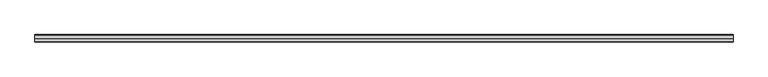
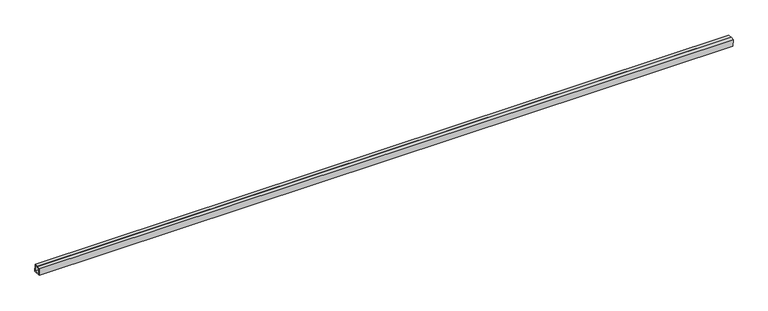
"""IFC4 building model written with IfcOpenShell, lengths in millimetres: proxy geometry, Inner panel:Inner panel:1:Inner panel:1 : Inner panel:Inner panel:300324:2:Inner panel:1:Inner panel:1 : Inner panel:Inner panel:300324:2 : Inner panel:Inner panel:1:Inner panel:1 : Inner panel:Inner panel:300324:300043:20 : Inner panel:Inner panel:1:Inner panel:1 : Inner panel:Inner panel:300324:2:Inner panel:1:Inner panel:1 : Inner panel:Inner panel:300324:2 : Inner panel:Inner panel:1:Inner panel:1 : Inner panel:Inner panel:300324:300043:308120."""

from ifc_helpers import new_model, si_unit, frame, origin, place, context, project, spatial, polyline, outline, extrude, source, transform, mapped, element, save


def generic_models_a2e03578(model_context):
    return source(origin(), model_context, "Body", "SweptSolid", [
        extrude(outline(polyline([(-569061.6758054, 8767.2361869), (-569043.4353822, 8767.9962045), (-569041.8492584, 8729.9292345), (-569079.9162285, 8728.3431107), (-569081.5023523, 8766.4100808), (-569063.2619291, 8767.1700984), (-569063.1627964, 8764.7909128), (-569079.0240339, 8764.1300279), (-569077.6361756, 8730.8214291), (-569044.3275768, 8732.2092874), (-569045.7154351, 8765.5178862), (-569061.5766726, 8764.8570013), (-569061.6758054, 8767.2361869)])), frame((593141.1867242, 0.0, 0.0), z_axis=(1.0, 0.0, 0.0), x_axis=(0.0, 1.0, 0.0)), (0.0, 0.0, 1.0), 3657.6),
    ])


if __name__ == "__main__":
    model = new_model("IFC4")
    model_context = context("Model", 3, world=origin())
    ifc_project = project(units=[si_unit("LENGTHUNIT", "METRE", prefix="MILLI")], contexts=[model_context])
    site = spatial("IfcSite", under=ifc_project)
    building = spatial("IfcBuilding", under=site)
    placement = place(None, origin())
    generic_models_shape = generic_models_a2e03578(model_context)
    element("IfcBuildingElementProxy", 1, Name="Inner panel:Inner panel:1:Inner panel:1 : Inner panel:Inner panel:300324:2:Inner panel:1:Inner panel:1 : Inner panel:Inner panel:300324:2 : Inner panel:Inner panel:1:Inner panel:1 : Inner panel:Inner panel:300324:300043:20 : Inner panel:Inner panel:1:Inner panel:1 : Inner panel:Inner panel:300324:2:Inner panel:1:Inner panel:1 : Inner panel:Inner panel:300324:2 : Inner panel:Inner panel:1:Inner panel:1 : Inner panel:Inner panel:300324:300043:308120", ObjectType="Inner panel:Inner panel:1:Inner panel:1 : Inner panel:Inner panel:300324:2:Inner panel:1:Inner panel:1 : Inner panel:Inner panel:300324:2 : Inner panel:Inner panel:1:Inner panel:1 : Inner panel:Inner panel:300324:300043:20 : Inner panel:Inner panel:1:Inner panel:1 : Inner panel:Inner panel:300324:2:Inner panel:1:Inner panel:1 : Inner panel:Inner panel:300324:2 : Inner panel:Inner panel:1:Inner panel:1 : Inner panel:Inner panel:300324:300043:308120", at=placement, inside=building, context=model_context, shape_type="MappedRepresentation", body=[
        mapped(generic_models_shape, transform((0.0, 0.0, 0.0), x_axis=(1.0, 0.0, 0.0), y_axis=(0.0, 1.0, 0.0), z_axis=(0.0, 0.0, 1.0))),
    ])
    save(model, "model.ifc")

# Revit data of these elements
# Type "Inner panel:Inner panel:1:Inner panel:1 : Inner panel:Inner panel:300324:2:Inner panel:1:Inner panel:1 : Inner panel:Inner panel:300324:2 : Inner panel:Inner panel:1:Inner panel:1 : Inner panel:Inner panel:300324:300043:20 : Inner panel:Inner panel:1:Inner panel:1 : Inner panel:Inner panel:300324:2:Inner panel:1:Inner panel:1 : Inner panel:Inner panel:300324:2 : Inner panel:Inner panel:1:Inner panel:1 : Inner panel:Inner panel:300324:300043:308120"
#   NameOverride = "Inner panel:Inner panel:1:Inner panel:1 : Inner panel:Inner panel:300324:2:Inner panel:1:Inner panel:1 : Inner panel:Inner panel:300324:2 : Inner panel:Inner panel:1:Inner panel:1 : Inner panel:Inner panel:300324:300043:308120"
#   ObjectTypeOverride = "Inner panel:1:Inner panel:1 : Inner panel:Inner panel:300324:2 : Inner panel:Inner panel:1:Inner panel:1 : Inner panel:Inner panel:300324:300043"
#   Reference = "Inner panel"
#   Tag = "308120"
# Element 1 (IfcBuildingElementProxy, "Inner panel:Inner panel:1:Inner panel:1 : Inner panel:Inner panel:300324:2:Inner panel:1:Inner panel:1 : Inner panel:Inner panel:300324:2 : Inner panel:Inner panel:1:Inner panel:1 : Inner panel:Inner panel:300324:300043:20 : Inner panel:Inner panel:1:Inner panel:1 : Inner panel:Inner panel:300324:2:Inner panel:1:Inner panel:1 : Inner panel:Inner panel:300324:2 : Inner panel:Inner panel:1:Inner panel:1 : Inner panel:Inner panel:300324:300043:308120")
#   Materials on its faces: "1 1/2\" X 1 1/2\" SPLIT-SEAM SQUARE TUBING (~24\" CANTILEVER FROM C.L. OF GLULAM)"
# Materials
#   "1 1/2\" X 1 1/2\" SPLIT-SEAM SQUARE TUBING (~24\" CANTILEVER FROM C.L. OF GLULAM)": class "Unassigned", colour RGB 202 201 200, transparency 0, Cost = 0
